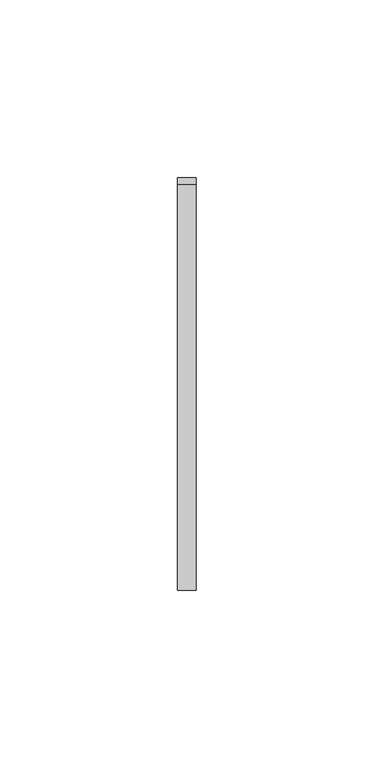
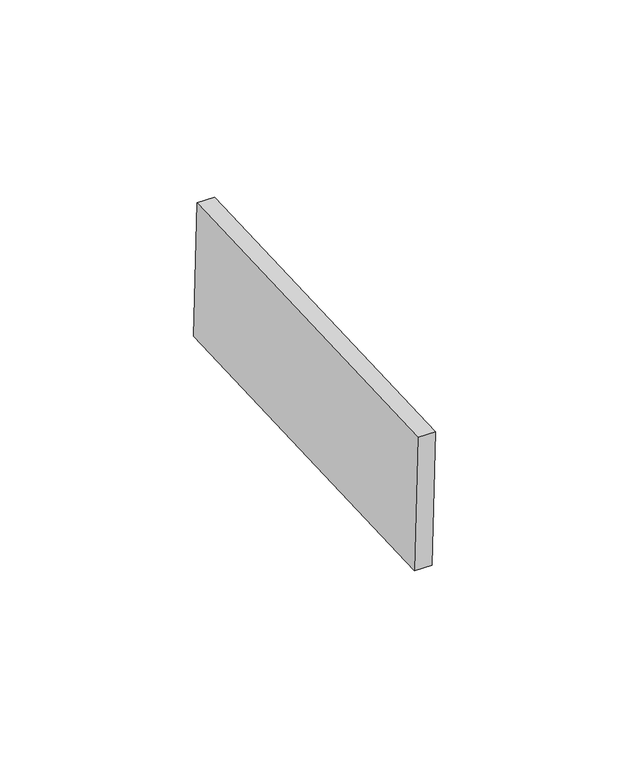
"""IFC4 building model written with IfcOpenShell, lengths in millimetres: proxy geometry, Inner panel:Inner panel:1:Inner panel:1 : Inner panel:Inner panel:300324:2:Inner panel:1:Inner panel:1 : Inner panel:Inner panel:300324:2 : Inner panel:Inner panel:1:Inner panel:1 : Inner panel:Inner panel:300324:300043:98 : Inner panel:Inner panel:1:Inner panel:1 : Inner panel:Inner panel:300324:2:Inner panel:1:Inner panel:1 : Inner panel:Inner panel:300324:2 : Inner panel:Inner panel:1:Inner panel:1 : Inner panel:Inner panel:300324:300043:308120."""

from ifc_helpers import new_model, si_unit, frame, origin, place, context, project, spatial, polyline, outline, extrude, source, transform, mapped, element, save


def generic_models_4f9416e8(model_context):
    return source(origin(), model_context, "Body", "SweptSolid", [
        extrude(outline(polyline([(0.0, -114.3), (0.0, 0.0), (5.2138089, 0.0), (5.2138089, -114.3), (0.0, -114.3)])), frame((593123.795117, -579007.2622385, 3952.103089), z_axis=(0.0, -0.04163054471216399, 0.9991330730923527), x_axis=(-1.0, 0.0, 0.0)), (0.0, 0.0, 1.0), 43.2233908),
    ])


if __name__ == "__main__":
    model = new_model("IFC4")
    model_context = context("Model", 3, world=origin())
    ifc_project = project(units=[si_unit("LENGTHUNIT", "METRE", prefix="MILLI")], contexts=[model_context])
    site = spatial("IfcSite", under=ifc_project)
    building = spatial("IfcBuilding", under=site)
    placement = place(None, origin())
    generic_models_shape = generic_models_4f9416e8(model_context)
    element("IfcBuildingElementProxy", 1, Name="Inner panel:Inner panel:1:Inner panel:1 : Inner panel:Inner panel:300324:2:Inner panel:1:Inner panel:1 : Inner panel:Inner panel:300324:2 : Inner panel:Inner panel:1:Inner panel:1 : Inner panel:Inner panel:300324:300043:98 : Inner panel:Inner panel:1:Inner panel:1 : Inner panel:Inner panel:300324:2:Inner panel:1:Inner panel:1 : Inner panel:Inner panel:300324:2 : Inner panel:Inner panel:1:Inner panel:1 : Inner panel:Inner panel:300324:300043:308120", ObjectType="Inner panel:Inner panel:1:Inner panel:1 : Inner panel:Inner panel:300324:2:Inner panel:1:Inner panel:1 : Inner panel:Inner panel:300324:2 : Inner panel:Inner panel:1:Inner panel:1 : Inner panel:Inner panel:300324:300043:98 : Inner panel:Inner panel:1:Inner panel:1 : Inner panel:Inner panel:300324:2:Inner panel:1:Inner panel:1 : Inner panel:Inner panel:300324:2 : Inner panel:Inner panel:1:Inner panel:1 : Inner panel:Inner panel:300324:300043:308120", at=placement, inside=building, context=model_context, shape_type="MappedRepresentation", body=[
        mapped(generic_models_shape, transform((0.0, 0.0, 0.0), x_axis=(1.0, 0.0, 0.0), y_axis=(0.0, 1.0, 0.0), z_axis=(0.0, 0.0, 1.0))),
    ])
    save(model, "model.ifc")

# Revit data of these elements
# Type "Inner panel:Inner panel:1:Inner panel:1 : Inner panel:Inner panel:300324:2:Inner panel:1:Inner panel:1 : Inner panel:Inner panel:300324:2 : Inner panel:Inner panel:1:Inner panel:1 : Inner panel:Inner panel:300324:300043:98 : Inner panel:Inner panel:1:Inner panel:1 : Inner panel:Inner panel:300324:2:Inner panel:1:Inner panel:1 : Inner panel:Inner panel:300324:2 : Inner panel:Inner panel:1:Inner panel:1 : Inner panel:Inner panel:300324:300043:308120"
#   NameOverride = "Inner panel:Inner panel:1:Inner panel:1 : Inner panel:Inner panel:300324:2:Inner panel:1:Inner panel:1 : Inner panel:Inner panel:300324:2 : Inner panel:Inner panel:1:Inner panel:1 : Inner panel:Inner panel:300324:300043:308120"
#   ObjectTypeOverride = "Inner panel:1:Inner panel:1 : Inner panel:Inner panel:300324:2 : Inner panel:Inner panel:1:Inner panel:1 : Inner panel:Inner panel:300324:300043"
#   Reference = "Inner panel"
#   Tag = "308120"
# Element 1 (IfcBuildingElementProxy, "Inner panel:Inner panel:1:Inner panel:1 : Inner panel:Inner panel:300324:2:Inner panel:1:Inner panel:1 : Inner panel:Inner panel:300324:2 : Inner panel:Inner panel:1:Inner panel:1 : Inner panel:Inner panel:300324:300043:98 : Inner panel:Inner panel:1:Inner panel:1 : Inner panel:Inner panel:300324:2:Inner panel:1:Inner panel:1 : Inner panel:Inner panel:300324:2 : Inner panel:Inner panel:1:Inner panel:1 : Inner panel:Inner panel:300324:300043:308120")
#   Materials on its faces: "SLIDING CLIP"
# Materials
#   "SLIDING CLIP": class "Generic", colour RGB 120 120 120, transparency 0, Cost = 0
